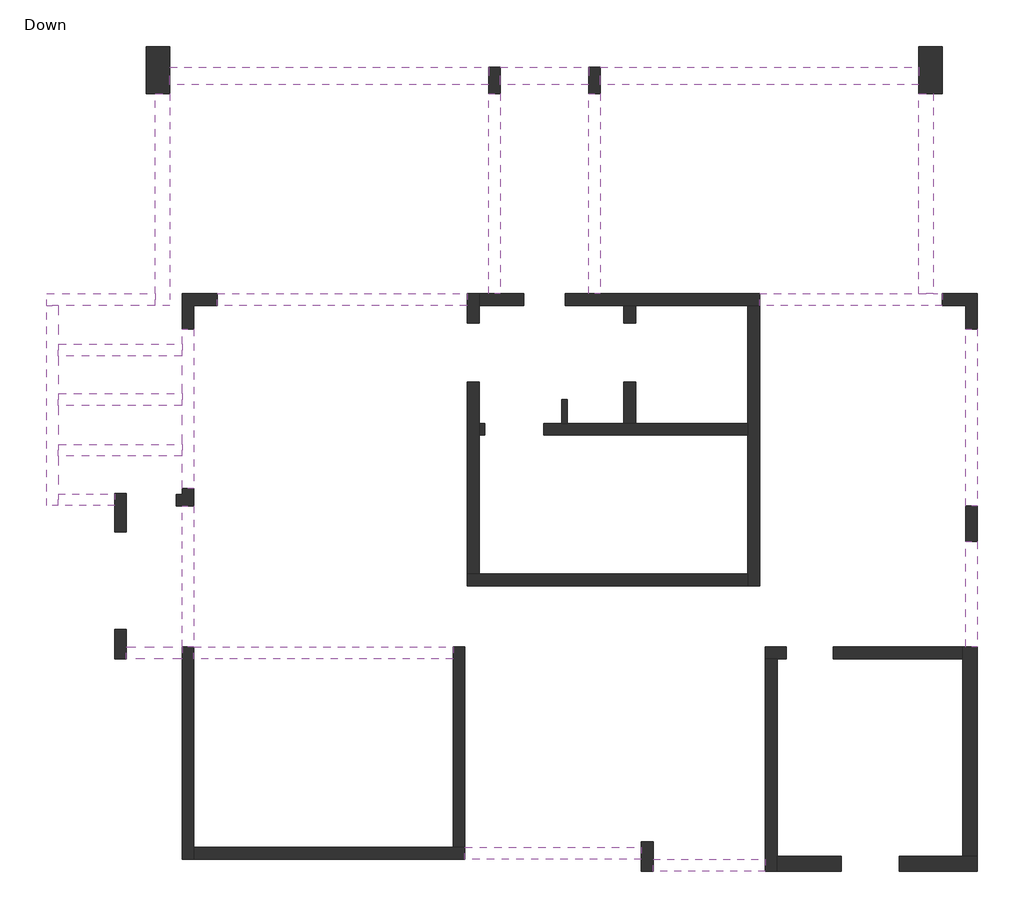
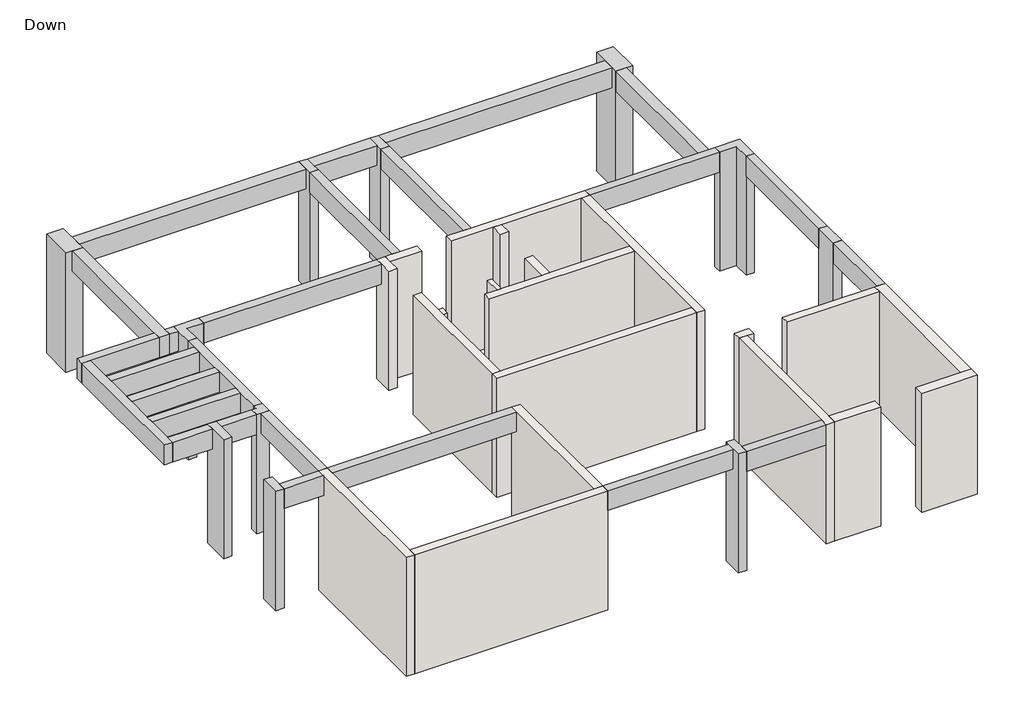
# One storey: 23 beams, 20 walls, 11 columns.
"""IFC4 building model written with IfcOpenShell, lengths in millimetres."""

from ifc_helpers import new_model, si_unit, frame, origin, origin_with_axes, place, context, project, spatial, polyline, outline, extrude, faceted_brep, element, save

model = new_model("IFC4")

# Units and contexts
model_context = context("Model", 3, world=origin())
ifc_project = project(units=[si_unit("LENGTHUNIT", "METRE", prefix="MILLI")], contexts=[model_context])

# Site, building, storey
site = spatial("IfcSite", under=ifc_project)
building = spatial("IfcBuilding", under=site)
storey = spatial("IfcBuildingStorey", under=building, Name="Down", Elevation=0.0)

# Beams
placement = place(None, origin())
element("IfcBeam", 1, ObjectType="Concrete Rectengular Beam : 20/50", at=placement, inside=storey, context=model_context, shape_type="Brep", body=[
    faceted_brep([(-4636.0027125, 7405.5532536, 3000.0), (-4636.0027125, 7605.5532536, 3000.0), (-8876.8844551, 7605.5532536, 3000.0), (-8876.8844551, 7405.5532536, 3000.0), (-4636.0027125, 7405.5532536, 2500.0), (-4636.0027125, 7405.5532536, 2850.0), (-8876.8844551, 7405.5532536, 2500.0), (-4636.0027125, 7605.5532536, 2500.0), (-8876.8844551, 7605.5532536, 2500.0)], [[[0, 1, 2, 3]], [[4, 5, 0, 3, 6]], [[7, 4, 6, 8]], [[1, 7, 8, 2]], [[1, 0, 5, 4, 7]], [[3, 2, 8, 6]]]),
])
element("IfcBeam", 2, ObjectType="Concrete Rectengular Beam : 20/50", at=placement, inside=storey, context=model_context, shape_type="Brep", body=[
    faceted_brep([(3423.240421, 7405.5532536, 3000.0), (3423.240421, 7605.5532536, 3000.0), (3276.9297982, 7605.5532536, 3000.0), (3026.9297982, 7605.5532536, 3000.0), (323.9972875, 7605.5532536, 3000.0), (323.9972875, 7405.5532536, 3000.0), (3423.240421, 7605.5532536, 2500.0), (3276.9297982, 7605.5532536, 2500.0), (3026.9297982, 7605.5532536, 2500.0), (323.9972875, 7605.5532536, 2500.0), (3423.240421, 7405.5532536, 2500.0), (323.9972875, 7405.5532536, 2500.0), (323.9972875, 7405.5532536, 2850.0)], [[[0, 1, 2, 3, 4, 5]], [[1, 6, 7, 8, 9, 4, 3, 2]], [[6, 10, 11, 9, 8, 7]], [[10, 0, 5, 12, 11]], [[1, 0, 10, 6]], [[5, 4, 9, 11, 12]]]),
])
element("IfcBeam", 3, ObjectType="Concrete Rectengular Beam : 20/50", at=placement, inside=storey, context=model_context, shape_type="Brep", body=[
    faceted_brep([(-9277.1472957, 1603.8855607, 3000.0), (-9277.1472957, 1403.8855607, 3000.0), (-4877.1268931, 1403.8855607, 3000.0), (-4877.1268931, 1603.8855607, 3000.0), (-9276.8844551, 1603.8855607, 3000.0), (-9277.1472957, 1603.8855607, 2500.0), (-4877.1268931, 1603.8855607, 2850.0), (-4877.1268931, 1603.8855607, 2500.0), (-9276.8844551, 1603.8855607, 2500.0), (-9277.1472957, 1403.8855607, 2500.0), (-4877.1268931, 1403.8855607, 2500.0), (-9277.1472957, 1403.8855607, 2850.0), (-4877.1268931, 1403.8855607, 2850.0)], [[[0, 1, 2, 3, 4]], [[5, 0, 4, 3, 6, 7, 8]], [[9, 5, 8, 7, 10]], [[1, 11, 9, 10, 12, 2]], [[1, 0, 5, 9, 11]], [[3, 2, 12, 10, 7, 6]]]),
])
element("IfcBeam", 4, ObjectType="Concrete Rectengular Beam : 20/50", at=placement, inside=storey, context=model_context, shape_type="Brep", body=[
    faceted_brep([(-9276.8844551, 3997.7532903, 3000.0), (-9476.8844551, 3997.7532903, 3000.0), (-9476.8844551, 1603.8855607, 3000.0), (-9277.1472957, 1603.8855607, 3000.0), (-9276.8844551, 1603.8855607, 3000.0), (-9276.8844551, 3997.7532903, 2500.0), (-9276.8844551, 1603.8855607, 2850.0), (-9276.8844551, 1603.8855607, 2500.0), (-9476.8844551, 3997.7532903, 2500.0), (-9277.1472957, 1603.8855607, 2500.0), (-9476.8844551, 1603.8855607, 2500.0), (-9476.8844551, 3997.7532903, 2850.0), (-9476.8844551, 1603.8855607, 2850.0)], [[[0, 1, 2, 3, 4]], [[5, 0, 4, 6, 7]], [[8, 5, 7, 9, 10]], [[1, 11, 8, 10, 12, 2]], [[1, 0, 5, 8, 11]], [[4, 3, 2, 12, 10, 9, 7, 6]]]),
])
element("IfcBeam", 5, ObjectType="Concrete Rectengular Beam : 20/50", at=placement, inside=storey, context=model_context, shape_type="Brep", body=[
    faceted_brep([(-9276.8844551, 7005.5532536, 3000.0), (-9476.8844551, 7005.5532536, 3000.0), (-9476.8844551, 6745.5532536, 3000.0), (-9476.8844551, 6545.5532536, 3000.0), (-9476.8844551, 5905.5532536, 3000.0), (-9476.8844551, 5705.5532536, 3000.0), (-9476.8844551, 5045.5532536, 3000.0), (-9476.8844551, 4845.5532536, 3000.0), (-9476.8844551, 4297.7532903, 3000.0), (-9276.8844551, 4297.7532903, 3000.0), (-9276.8844551, 7005.5532536, 2500.0), (-9276.8844551, 4297.7532903, 2500.0), (-9476.8844551, 7005.5532536, 2500.0), (-9476.8844551, 4297.7532903, 2500.0), (-9476.8844551, 4845.5532536, 2500.0), (-9476.8844551, 5045.5532536, 2500.0), (-9476.8844551, 5705.5532536, 2500.0), (-9476.8844551, 5905.5532536, 2500.0), (-9476.8844551, 6545.5532536, 2500.0), (-9476.8844551, 6745.5532536, 2500.0)], [[[0, 1, 2, 3, 4, 5, 6, 7, 8, 9]], [[10, 0, 9, 11]], [[12, 10, 11, 13, 14, 15, 16, 17, 18, 19]], [[1, 12, 19, 18, 17, 16, 15, 14, 13, 8, 7, 6, 5, 4, 3, 2]], [[1, 0, 10, 12]], [[9, 8, 13, 11]]]),
])
element("IfcBeam", 6, ObjectType="Concrete Rectengular Beam : 20/50", at=placement, inside=storey, context=model_context, shape_type="Brep", body=[
    faceted_brep([(-1681.0647566, -1997.4530794, 3000.0), (-1681.0647566, -1797.4530794, 3000.0), (-4677.1268931, -1797.4530794, 3000.0), (-4677.1268931, -1997.4530794, 3000.0), (-1681.0647566, -1997.4530794, 2500.0), (-4677.1268931, -1997.4530794, 2500.0), (-1681.0647566, -1797.4530794, 2500.0), (-4677.1268931, -1797.4530794, 2500.0), (-1681.0647566, -1797.4530794, 2850.0), (-4677.1268931, -1797.4530794, 2850.0)], [[[0, 1, 2, 3]], [[4, 0, 3, 5]], [[6, 4, 5, 7]], [[2, 1, 8, 6, 7, 9]], [[1, 0, 4, 6, 8]], [[3, 2, 9, 7, 5]]]),
])
element("IfcBeam", 7, ObjectType="Concrete Rectengular Beam : 20/50", at=placement, inside=storey, context=model_context, shape_type="Brep", body=[
    faceted_brep([(-1481.0647566, -2001.586272, 3000.0), (-1481.0647566, -2201.586272, 3000.0), (423.0052446, -2201.586272, 3000.0), (423.0052446, -2001.586272, 3000.0), (-1481.0647566, -2201.586272, 2500.0), (423.0052446, -2201.586272, 2500.0), (-1481.0647566, -2001.586272, 2500.0), (423.0052446, -2001.586272, 2500.0), (-1481.0647566, -2001.586272, 2850.0), (423.0052446, -2001.586272, 2850.0)], [[[0, 1, 2, 3]], [[1, 4, 5, 2]], [[4, 6, 7, 5]], [[6, 8, 0, 3, 9, 7]], [[1, 0, 8, 6, 4]], [[3, 2, 5, 7, 9]]]),
])
element("IfcBeam", 8, ObjectType="Concrete Rectengular Beam : 20/50", at=placement, inside=storey, context=model_context, shape_type="Brep", body=[
    faceted_brep([(4023.240421, 3398.9311809, 3000.0), (3823.240421, 3398.9311809, 3000.0), (3823.240421, 1603.8858088, 3000.0), (4023.240421, 1603.8858088, 3000.0), (4023.240421, 3398.9311809, 2500.0), (4023.240421, 1603.8858088, 2500.0), (3823.240421, 3398.9311809, 2500.0), (3823.240421, 1603.8858088, 2500.0), (3823.240421, 1603.8858088, 2850.0)], [[[0, 1, 2, 3]], [[4, 0, 3, 5]], [[6, 4, 5, 7]], [[1, 6, 7, 8, 2]], [[1, 0, 4, 6]], [[3, 2, 8, 7, 5]]]),
])
element("IfcBeam", 9, ObjectType="Concrete Rectengular Beam : 20/50", at=placement, inside=storey, context=model_context, shape_type="SweptSolid", body=[
    extrude(outline(polyline([(3823.240421, 7005.5532536), (4023.240421, 7005.5532536), (4023.240421, 3998.9311809), (3823.240421, 3998.9311809), (3823.240421, 7005.5532536)])), frame((0.0, 0.0, 2500.0), z_axis=(0.0, 0.0, 1.0), x_axis=(1.0, 0.0, 0.0)), (0.0, 0.0, 1.0), 500.0),
])
element("IfcBeam", 10, ObjectType="Concrete Rectengular Beam : 20/50", at=placement, inside=storey, context=model_context, shape_type="Brep", body=[
    faceted_brep([(-2375.600893, 11003.3317688, 3000.0), (-2575.600893, 11003.3317688, 3000.0), (-2575.600893, 7605.5532536, 3000.0), (-2375.600893, 7605.5532536, 3000.0), (-2575.600893, 11003.3317688, 2500.0), (-2575.600893, 7605.5532536, 2500.0), (-2575.600893, 7605.5532536, 2850.0), (-2375.600893, 11003.3317688, 2500.0), (-2375.600893, 7605.5532536, 2500.0), (-2375.600893, 7605.5532536, 2850.0)], [[[0, 1, 2, 3]], [[1, 4, 5, 6, 2]], [[4, 7, 8, 5]], [[7, 0, 3, 9, 8]], [[1, 0, 7, 4]], [[3, 2, 6, 5, 8, 9]]]),
])
element("IfcBeam", 11, ObjectType="Concrete Rectengular Beam : 20/50", at=placement, inside=storey, context=model_context, shape_type="Brep", body=[
    faceted_brep([(-4072.3731245, 11003.3317688, 3000.0), (-4272.3731245, 11003.3317688, 3000.0), (-4272.3731245, 7605.5532536, 3000.0), (-4072.3731245, 7605.5532536, 3000.0), (-4072.3731245, 11003.3317688, 2500.0), (-4072.3731245, 7605.5532536, 2850.0), (-4072.3731245, 7605.5532536, 2500.0), (-4272.3731245, 11003.3317688, 2500.0), (-4272.3731245, 7605.5532536, 2500.0), (-4272.3731245, 7605.5532536, 2850.0)], [[[0, 1, 2, 3]], [[4, 0, 3, 5, 6]], [[7, 4, 6, 8]], [[1, 7, 8, 9, 2]], [[1, 0, 4, 7]], [[3, 2, 9, 8, 6, 5]]]),
])
element("IfcBeam", 12, ObjectType="Concrete Rectengular Beam : 20/50", at=placement, inside=storey, context=model_context, shape_type="Brep", body=[
    faceted_brep([(-9476.8844551, 7405.5532536, 3000.0), (-9476.8844551, 7605.5532536, 3000.0), (-9682.6961091, 7605.5532536, 3000.0), (-9682.6961091, 7405.5532536, 3000.0), (-9476.8844551, 7605.5532536, 2500.0), (-9682.6961091, 7605.5532536, 2500.0), (-9682.6961091, 7605.5532536, 2850.0), (-9476.8844551, 7405.5532536, 2500.0), (-9682.6961091, 7405.5532536, 2500.0), (-9476.8844551, 7405.5532536, 2850.0)], [[[0, 1, 2, 3]], [[1, 4, 5, 6, 2]], [[4, 7, 8, 5]], [[7, 9, 0, 3, 8]], [[1, 0, 9, 7, 4]], [[3, 2, 6, 5, 8]]]),
    faceted_brep([(-11776.8844551, 7405.5532536, 3000.0), (-11776.8844551, 7605.5532536, 3000.0), (-11776.8844551, 7605.5532536, 2500.0), (-11776.8844551, 7405.5532536, 2500.0), (-9932.6961091, 7605.5532536, 3000.0), (-9932.6961091, 7405.5532536, 3000.0), (-9932.6961091, 7405.5532536, 2500.0), (-9932.6961091, 7605.5532536, 2500.0), (-11576.8844551, 7405.5532536, 3000.0), (-11576.8844551, 7405.5532536, 2500.0)], [[[0, 1, 2, 3]], [[4, 5, 6, 7]], [[1, 0, 8, 5, 4]], [[2, 1, 4, 7]], [[3, 2, 7, 6, 9]], [[0, 3, 9, 6, 5, 8]]]),
])
element("IfcBeam", 13, ObjectType="Concrete Rectengular Beam : 20/50", at=placement, inside=storey, context=model_context, shape_type="Brep", body=[
    faceted_brep([(-11776.8844551, 4005.5532536, 3000.0), (-11576.8844551, 4005.5532536, 3000.0), (-11576.8844551, 4205.5532536, 3000.0), (-11576.8844551, 4845.5532536, 3000.0), (-11576.8844551, 5045.5532536, 3000.0), (-11576.8844551, 5705.5532536, 3000.0), (-11576.8844551, 5905.5532536, 3000.0), (-11576.8844551, 6545.5532536, 3000.0), (-11576.8844551, 6745.5532536, 3000.0), (-11576.8844551, 7405.5532536, 3000.0), (-11776.8844551, 7405.5532536, 3000.0), (-11776.8844551, 4005.5532536, 2500.0), (-11776.8844551, 7405.5532536, 2500.0), (-11576.8844551, 4005.5532536, 2500.0), (-11576.8844551, 7405.5532536, 2500.0), (-11576.8844551, 6745.5532536, 2500.0), (-11576.8844551, 6545.5532536, 2500.0), (-11576.8844551, 5905.5532536, 2500.0), (-11576.8844551, 5705.5532536, 2500.0), (-11576.8844551, 5045.5532536, 2500.0), (-11576.8844551, 4845.5532536, 2500.0), (-11576.8844551, 4205.5532536, 2500.0), (-11576.8844551, 7405.5532536, 2850.0)], [[[0, 1, 2, 3, 4, 5, 6, 7, 8, 9, 10]], [[11, 0, 10, 12]], [[13, 11, 12, 14, 15, 16, 17, 18, 19, 20, 21]], [[1, 13, 21, 20, 19, 18, 17, 16, 15, 14, 22, 9, 8, 7, 6, 5, 4, 3, 2]], [[10, 9, 22, 14, 12]], [[1, 0, 11, 13]]]),
])
element("IfcBeam", 14, ObjectType="Concrete Rectengular Beam : 20/50", at=placement, inside=storey, context=model_context, shape_type="Brep", body=[
    faceted_brep([(-9576.8844551, 4005.5532536, 3000.0), (-9576.8844551, 4197.7532903, 3000.0), (-9476.8844551, 4197.7532903, 3000.0), (-9476.8844551, 4205.5532536, 3000.0), (-10423.025528, 4205.5532536, 3000.0), (-10423.025528, 4005.5532536, 3000.0), (-9576.8844551, 4005.5532536, 2500.0), (-9576.8844551, 4005.5532536, 2850.0), (-10423.025528, 4005.5532536, 2850.0), (-10423.025528, 4005.5532536, 2500.0), (-9576.8844551, 4197.7532903, 2500.0), (-10423.025528, 4205.5532536, 2500.0), (-9476.8844551, 4205.5532536, 2500.0), (-9476.8844551, 4197.7532903, 2500.0), (-9476.8844551, 4205.5532536, 2850.0), (-10423.025528, 4205.5532536, 2850.0)], [[[0, 1, 2, 3, 4, 5]], [[6, 7, 0, 5, 8, 9]], [[10, 6, 9, 11, 12, 13]], [[3, 14, 12, 11, 15, 4]], [[10, 1, 0, 7, 6]], [[1, 10, 13, 2]], [[2, 13, 12, 14, 3]], [[5, 4, 15, 11, 9, 8]]]),
    faceted_brep([(-11576.8844551, 4005.5532536, 3000.0), (-11576.8844551, 4205.5532536, 3000.0), (-11576.8844551, 4205.5532536, 2850.0), (-11576.8844551, 4205.5532536, 2500.0), (-11576.8844551, 4005.5532536, 2500.0), (-10623.025528, 4205.5532536, 3000.0), (-10623.025528, 4005.5532536, 3000.0), (-10623.025528, 4005.5532536, 2500.0), (-10623.025528, 4205.5532536, 2500.0), (-10623.025528, 4205.5532536, 2850.0)], [[[0, 1, 2, 3, 4]], [[5, 6, 7, 8, 9]], [[1, 0, 6, 5]], [[0, 4, 7, 6]], [[4, 3, 8, 7]], [[3, 2, 1, 5, 9, 8]]]),
])
element("IfcBeam", 15, ObjectType="Concrete Rectengular Beam : 20/50", at=placement, inside=storey, context=model_context, shape_type="Brep", body=[
    faceted_brep([(-9476.8844551, 4845.5532536, 3000.0), (-9476.8844551, 5045.5532536, 3000.0), (-11576.8844551, 5045.5532536, 3000.0), (-11576.8844551, 4845.5532536, 3000.0), (-9476.8844551, 5045.5532536, 2850.0), (-9476.8844551, 5045.5532536, 2500.0), (-11576.8844551, 5045.5532536, 2500.0), (-11576.8844551, 5045.5532536, 2850.0), (-9476.8844551, 4845.5532536, 2500.0), (-11576.8844551, 4845.5532536, 2500.0), (-9476.8844551, 4845.5532536, 2850.0), (-11576.8844551, 4845.5532536, 2850.0)], [[[0, 1, 2, 3]], [[1, 4, 5, 6, 7, 2]], [[5, 8, 9, 6]], [[8, 10, 0, 3, 11, 9]], [[1, 0, 10, 8, 5, 4]], [[3, 2, 7, 6, 9, 11]]]),
])
element("IfcBeam", 16, ObjectType="Concrete Rectengular Beam : 20/50", at=placement, inside=storey, context=model_context, shape_type="Brep", body=[
    faceted_brep([(-9476.8844551, 5705.5532536, 3000.0), (-9476.8844551, 5905.5532536, 3000.0), (-11576.8844551, 5905.5532536, 3000.0), (-11576.8844551, 5705.5532536, 3000.0), (-9476.8844551, 5905.5532536, 2850.0), (-9476.8844551, 5905.5532536, 2500.0), (-11576.8844551, 5905.5532536, 2500.0), (-11576.8844551, 5905.5532536, 2850.0), (-9476.8844551, 5705.5532536, 2500.0), (-11576.8844551, 5705.5532536, 2500.0), (-9476.8844551, 5705.5532536, 2850.0), (-11576.8844551, 5705.5532536, 2850.0)], [[[0, 1, 2, 3]], [[1, 4, 5, 6, 7, 2]], [[5, 8, 9, 6]], [[8, 10, 0, 3, 11, 9]], [[1, 0, 10, 8, 5, 4]], [[3, 2, 7, 6, 9, 11]]]),
])
element("IfcBeam", 17, ObjectType="Concrete Rectengular Beam : 20/50", at=placement, inside=storey, context=model_context, shape_type="Brep", body=[
    faceted_brep([(-9476.8844551, 6545.5532536, 3000.0), (-9476.8844551, 6745.5532536, 3000.0), (-11576.8844551, 6745.5532536, 3000.0), (-11576.8844551, 6545.5532536, 3000.0), (-9476.8844551, 6745.5532536, 2850.0), (-9476.8844551, 6745.5532536, 2500.0), (-11576.8844551, 6745.5532536, 2500.0), (-11576.8844551, 6745.5532536, 2850.0), (-9476.8844551, 6545.5532536, 2500.0), (-11576.8844551, 6545.5532536, 2500.0), (-9476.8844551, 6545.5532536, 2850.0), (-11576.8844551, 6545.5532536, 2850.0)], [[[0, 1, 2, 3]], [[1, 4, 5, 6, 7, 2]], [[5, 8, 9, 6]], [[8, 10, 0, 3, 11, 9]], [[1, 0, 10, 8, 5, 4]], [[3, 2, 7, 6, 9, 11]]]),
])
element("IfcBeam", 18, ObjectType="Concrete Rectengular Beam : 20/50", at=placement, inside=storey, context=model_context, shape_type="Brep", body=[
    faceted_brep([(-10423.025528, 1603.8855607, 3000.0), (-10423.025528, 1403.8855607, 3000.0), (-9477.1472957, 1403.8855607, 3000.0), (-9477.1472957, 1603.8855607, 3000.0), (-10423.025528, 1603.8855607, 2500.0), (-10423.025528, 1603.8855607, 2850.0), (-9477.1472957, 1603.8855607, 2500.0), (-10423.025528, 1403.8855607, 2500.0), (-9477.1472957, 1403.8855607, 2500.0)], [[[0, 1, 2, 3]], [[4, 5, 0, 3, 6]], [[7, 4, 6, 8]], [[1, 7, 8, 2]], [[1, 0, 5, 4, 7]], [[3, 2, 8, 6]]]),
])
element("IfcBeam", 19, ObjectType="Concrete Rectengular Beam : 25/50", at=placement, inside=storey, context=model_context, shape_type="Brep", body=[
    faceted_brep([(3276.9297982, 11001.5732233, 3000.0), (3026.9297982, 11001.5732233, 3000.0), (3026.9297982, 7605.5532536, 3000.0), (3276.9297982, 7605.5532536, 3000.0), (3276.9297982, 11001.5732233, 2500.0), (3276.9297982, 7605.5532536, 2500.0), (3026.9297982, 11001.5732233, 2500.0), (3026.9297982, 7605.5532536, 2500.0), (3026.9297982, 7605.5532536, 2850.0)], [[[0, 1, 2, 3]], [[4, 0, 3, 5]], [[6, 4, 5, 7]], [[1, 6, 7, 8, 2]], [[1, 0, 4, 6]], [[3, 2, 8, 7, 5]]]),
])
element("IfcBeam", 20, ObjectType="Concrete Rectengular Beam : 25/50", at=placement, inside=storey, context=model_context, shape_type="Brep", body=[
    faceted_brep([(-9932.6961091, 7405.5532536, 3000.0), (-9682.6961091, 7405.5532536, 3000.0), (-9682.6961091, 7605.5532536, 3000.0), (-9682.6961091, 11001.5732233, 3000.0), (-9932.6961091, 11001.5732233, 3000.0), (-9932.6961091, 7605.5532536, 3000.0), (-9682.6961091, 7405.5532536, 2500.0), (-9682.6961091, 7605.5532536, 2500.0), (-9682.6961091, 11001.5732233, 2500.0), (-9932.6961091, 7405.5532536, 2500.0), (-9932.6961091, 7605.5532536, 2500.0), (-9932.6961091, 11001.5732233, 2500.0)], [[[0, 1, 2, 3, 4, 5]], [[1, 6, 7, 8, 3, 2]], [[6, 9, 10, 11, 8, 7]], [[9, 0, 5, 4, 11, 10]], [[4, 3, 8, 11]], [[1, 0, 9, 6]]]),
])
element("IfcBeam", 21, ObjectType="Concrete Rectengular Beam : 30/50", at=placement, inside=storey, context=model_context, shape_type="Brep", body=[
    faceted_brep([(-9682.6961091, 11451.9234339, 3000.0), (-9682.6961091, 11151.9234339, 3000.0), (-4272.3731245, 11151.9234339, 3000.0), (-4272.3731245, 11451.9234339, 3000.0), (-9682.6961091, 11451.9234339, 2500.0), (-4272.3731245, 11451.9234339, 2500.0), (-9682.6961091, 11151.9234339, 2500.0), (-4272.3731245, 11151.9234339, 2500.0), (-9682.6961091, 11151.9234339, 2850.0), (-4272.3731245, 11151.9234339, 2850.0)], [[[0, 1, 2, 3]], [[4, 0, 3, 5]], [[6, 4, 5, 7]], [[1, 8, 6, 7, 9, 2]], [[1, 0, 4, 6, 8]], [[3, 2, 9, 7, 5]]]),
])
element("IfcBeam", 22, ObjectType="Concrete Rectengular Beam : 30/50", at=placement, inside=storey, context=model_context, shape_type="Brep", body=[
    faceted_brep([(-2575.600893, 11151.9234339, 3000.0), (-2575.600893, 11451.9234339, 3000.0), (-4072.3731245, 11451.9234339, 3000.0), (-4072.3731245, 11151.9234339, 3000.0), (-2575.600893, 11151.9234339, 2500.0), (-2575.600893, 11151.9234339, 2850.0), (-4072.3731245, 11151.9234339, 2850.0), (-4072.3731245, 11151.9234339, 2500.0), (-2575.600893, 11451.9234339, 2500.0), (-4072.3731245, 11451.9234339, 2500.0)], [[[0, 1, 2, 3]], [[4, 5, 0, 3, 6, 7]], [[8, 4, 7, 9]], [[1, 8, 9, 2]], [[1, 0, 5, 4, 8]], [[3, 2, 9, 7, 6]]]),
])
element("IfcBeam", 23, ObjectType="Concrete Rectengular Beam : 30/50", at=placement, inside=storey, context=model_context, shape_type="Brep", body=[
    faceted_brep([(3026.9297982, 11151.9234339, 3000.0), (3026.9297982, 11451.9234339, 3000.0), (-2375.600893, 11451.9234339, 3000.0), (-2375.600893, 11151.9234339, 3000.0), (3026.9297982, 11151.9234339, 2500.0), (3026.9297982, 11151.9234339, 2850.0), (-2375.600893, 11151.9234339, 2850.0), (-2375.600893, 11151.9234339, 2500.0), (3026.9297982, 11451.9234339, 2500.0), (-2375.600893, 11451.9234339, 2500.0)], [[[0, 1, 2, 3]], [[4, 5, 0, 3, 6, 7]], [[8, 4, 7, 9]], [[1, 8, 9, 2]], [[1, 0, 5, 4, 8]], [[3, 2, 9, 7, 6]]]),
])

# Columns
element("IfcColumn", 24, ObjectType="Concrete Rectengular Column : 20/45", at=placement, inside=storey, context=model_context, shape_type="Brep", body=[
    faceted_brep([(-2375.600893, 11453.3317688, 0.0), (-2375.600893, 11003.3317688, 0.0), (-2575.600893, 11003.3317688, 0.0), (-2575.600893, 11453.3317688, 0.0), (-2375.600893, 11453.3317688, 3000.0), (-2375.600893, 11151.9234339, 3000.0), (-2375.600893, 11003.3317688, 3000.0), (-2575.600893, 11003.3317688, 3000.0), (-2575.600893, 11151.9234339, 3000.0), (-2575.600893, 11453.3317688, 3000.0)], [[[0, 1, 2, 3]], [[4, 5, 6, 1, 0]], [[6, 7, 2, 1]], [[7, 8, 9, 3, 2]], [[9, 4, 0, 3]], [[4, 9, 8, 7, 6, 5]]]),
])
element("IfcColumn", 25, ObjectType="Concrete Rectengular Column : 20/45", at=placement, inside=storey, context=model_context, shape_type="Brep", body=[
    faceted_brep([(-4072.3731245, 11453.3317688, 0.0), (-4072.3731245, 11003.3317688, 0.0), (-4272.3731245, 11003.3317688, 0.0), (-4272.3731245, 11453.3317688, 0.0), (-4072.3731245, 11453.3317688, 3000.0), (-4072.3731245, 11151.9234339, 3000.0), (-4072.3731245, 11003.3317688, 3000.0), (-4272.3731245, 11003.3317688, 3000.0), (-4272.3731245, 11151.9234339, 3000.0), (-4272.3731245, 11453.3317688, 3000.0)], [[[0, 1, 2, 3]], [[4, 5, 6, 1, 0]], [[6, 7, 2, 1]], [[7, 8, 9, 3, 2]], [[9, 4, 0, 3]], [[4, 9, 8, 7, 6, 5]]]),
])
element("IfcColumn", 26, ObjectType="Concrete Rectengular Column : 20/50", at=placement, inside=storey, context=model_context, shape_type="Brep", body=[
    faceted_brep([(-10423.025528, 1900.4395709, 0.0), (-10423.025528, 1400.4395709, 0.0), (-10623.025528, 1400.4395709, 0.0), (-10623.025528, 1900.4395709, 0.0), (-10423.025528, 1900.4395709, 3000.0), (-10423.025528, 1603.8855607, 3000.0), (-10423.025528, 1400.4395709, 3000.0), (-10423.025528, 1900.4395709, 2850.0), (-10623.025528, 1400.4395709, 3000.0), (-10623.025528, 1900.4395709, 3000.0), (-10623.025528, 1900.4395709, 2850.0)], [[[0, 1, 2, 3]], [[4, 5, 6, 1, 0, 7]], [[6, 8, 2, 1]], [[8, 9, 10, 3, 2]], [[9, 4, 7, 0, 3, 10]], [[4, 9, 8, 6, 5]]]),
])
element("IfcColumn", 27, ObjectType="Concrete Rectengular Column : 20/50", at=placement, inside=storey, context=model_context, shape_type="Brep", body=[
    faceted_brep([(-1481.0647566, -1701.586272, 0.0), (-1481.0647566, -2201.586272, 0.0), (-1681.0647566, -2201.586272, 0.0), (-1681.0647566, -1701.586272, 0.0), (-1481.0647566, -1701.586272, 3000.0), (-1481.0647566, -2001.586272, 3000.0), (-1481.0647566, -2201.586272, 3000.0), (-1481.0647566, -1701.586272, 2850.0), (-1681.0647566, -2201.586272, 3000.0), (-1681.0647566, -1797.4530794, 3000.0), (-1681.0647566, -1701.586272, 3000.0), (-1681.0647566, -1701.586272, 2850.0)], [[[0, 1, 2, 3]], [[4, 5, 6, 1, 0, 7]], [[6, 8, 2, 1]], [[8, 9, 10, 11, 3, 2]], [[10, 4, 7, 0, 3, 11]], [[4, 10, 9, 8, 6, 5]]]),
])
element("IfcColumn", 28, ObjectType="Concrete Rectengular Column : 20/60", at=placement, inside=storey, context=model_context, shape_type="SweptSolid", body=[
    extrude(outline(polyline([(4023.240421, 3998.9311809), (4023.240421, 3398.9311809), (3823.240421, 3398.9311809), (3823.240421, 3998.9311809), (4023.240421, 3998.9311809)])), origin_with_axes(), (0.0, 0.0, 1.0), 3000.0),
])
element("IfcColumn", 29, ObjectType="Concrete Rectengular Column : 20/65", at=placement, inside=storey, context=model_context, shape_type="Brep", body=[
    faceted_brep([(-10423.025528, 4208.1905626, 0.0), (-10423.025528, 3558.1905626, 0.0), (-10623.025528, 3558.1905626, 0.0), (-10623.025528, 4208.1905626, 0.0), (-10423.025528, 4208.1905626, 3000.0), (-10423.025528, 4205.5532536, 3000.0), (-10423.025528, 4005.5532536, 3000.0), (-10423.025528, 3558.1905626, 3000.0), (-10423.025528, 3558.1905626, 2850.0), (-10423.025528, 4208.1905626, 2850.0), (-10623.025528, 3558.1905626, 3000.0), (-10623.025528, 3558.1905626, 2850.0), (-10623.025528, 4005.5532536, 3000.0), (-10623.025528, 4205.5532536, 3000.0), (-10623.025528, 4208.1905626, 3000.0), (-10623.025528, 4208.1905626, 2850.0)], [[[0, 1, 2, 3]], [[4, 5, 6, 7, 8, 1, 0, 9]], [[7, 10, 11, 2, 1, 8]], [[10, 12, 13, 14, 15, 3, 2, 11]], [[14, 4, 9, 0, 3, 15]], [[4, 14, 13, 12, 10, 7, 6, 5]]]),
])
element("IfcColumn", 30, ObjectType="Concrete Rectengular Column : 40/80", at=placement, inside=storey, context=model_context, shape_type="Brep", body=[
    faceted_brep([(3426.9297982, 11801.5732233, 0.0), (3426.9297982, 11001.5732233, 0.0), (3026.9297982, 11001.5732233, 0.0), (3026.9297982, 11801.5732233, 0.0), (3426.9297982, 11801.5732233, 3000.0), (3426.9297982, 11001.5732233, 3000.0), (3026.9297982, 11001.5732233, 3000.0), (3026.9297982, 11151.9234339, 3000.0), (3026.9297982, 11801.5732233, 3000.0)], [[[0, 1, 2, 3]], [[4, 5, 1, 0]], [[5, 6, 2, 1]], [[6, 7, 8, 3, 2]], [[8, 4, 0, 3]], [[4, 8, 7, 6, 5]]]),
])
element("IfcColumn", 31, ObjectType="Concrete Rectengular Column : 40/80", at=placement, inside=storey, context=model_context, shape_type="Brep", body=[
    faceted_brep([(-9682.6961091, 11801.5732233, 0.0), (-9682.6961091, 11001.5732233, 0.0), (-10082.6961091, 11001.5732233, 0.0), (-10082.6961091, 11801.5732233, 0.0), (-9682.6961091, 11801.5732233, 3000.0), (-9682.6961091, 11151.9234339, 3000.0), (-9682.6961091, 11001.5732233, 3000.0), (-10082.6961091, 11001.5732233, 3000.0), (-10082.6961091, 11801.5732233, 3000.0)], [[[0, 1, 2, 3]], [[4, 5, 6, 1, 0]], [[6, 7, 2, 1]], [[7, 8, 3, 2]], [[8, 4, 0, 3]], [[4, 8, 7, 6, 5]]]),
])
element("IfcColumn", 32, ObjectType="L Column : 30/30/20/20", at=placement, inside=storey, context=model_context, shape_type="Brep", body=[
    faceted_brep([(-9276.8844551, 3997.7532903, 0.0), (-9576.8844551, 3997.7532903, 0.0), (-9576.8844551, 4197.7532903, 0.0), (-9476.8844551, 4197.7532903, 0.0), (-9476.8844551, 4297.7532903, 0.0), (-9276.8844551, 4297.7532903, 0.0), (-9276.8844551, 3997.7532903, 3000.0), (-9476.8844551, 3997.7532903, 3000.0), (-9576.8844551, 3997.7532903, 3000.0), (-9576.8844551, 3997.7532903, 2850.0), (-9576.8844551, 4005.5532536, 3000.0), (-9576.8844551, 4197.7532903, 3000.0), (-9476.8844551, 4197.7532903, 3000.0), (-9476.8844551, 4205.5532536, 3000.0), (-9476.8844551, 4297.7532903, 3000.0), (-9276.8844551, 4297.7532903, 3000.0)], [[[0, 1, 2, 3, 4, 5]], [[6, 7, 8, 9, 1, 0]], [[8, 10, 11, 2, 1, 9]], [[11, 12, 3, 2]], [[12, 13, 14, 4, 3]], [[14, 15, 5, 4]], [[15, 6, 0, 5]], [[6, 15, 14, 13, 12, 11, 10, 8, 7]]]),
])
element("IfcColumn", 33, ObjectType="L Column : 60/60/20/20", at=placement, inside=storey, context=model_context, shape_type="Brep", body=[
    faceted_brep([(4023.240421, 7605.5532536, 0.0), (4023.240421, 7005.5532536, 0.0), (3823.240421, 7005.5532536, 0.0), (3823.240421, 7405.5532536, 0.0), (3423.240421, 7405.5532536, 0.0), (3423.240421, 7605.5532536, 0.0), (4023.240421, 7605.5532536, 3000.0), (4023.240421, 7005.5532536, 3000.0), (3823.240421, 7005.5532536, 3000.0), (3823.240421, 7405.5532536, 3000.0), (3823.240421, 7405.5532536, 2850.0), (3423.240421, 7405.5532536, 3000.0), (3423.240421, 7605.5532536, 3000.0)], [[[0, 1, 2, 3, 4, 5]], [[6, 7, 1, 0]], [[7, 8, 2, 1]], [[8, 9, 10, 3, 2]], [[9, 11, 4, 3, 10]], [[11, 12, 5, 4]], [[12, 6, 0, 5]], [[6, 12, 11, 9, 8, 7]]]),
])
element("IfcColumn", 34, ObjectType="L Column : 60/60/20/20", at=placement, inside=storey, context=model_context, shape_type="Brep", body=[
    faceted_brep([(-9476.8844551, 7605.5532536, 0.0), (-8876.8844551, 7605.5532536, 0.0), (-8876.8844551, 7405.5532536, 0.0), (-9276.8844551, 7405.5532536, 0.0), (-9276.8844551, 7005.5532536, 0.0), (-9476.8844551, 7005.5532536, 0.0), (-9476.8844551, 7605.5532536, 3000.0), (-8876.8844551, 7605.5532536, 3000.0), (-8876.8844551, 7605.5532536, 2500.0), (-8876.8844551, 7405.5532536, 3000.0), (-8876.8844551, 7405.5532536, 2500.0), (-9276.8844551, 7405.5532536, 3000.0), (-9276.8844551, 7405.5532536, 2850.0), (-9276.8844551, 7005.5532536, 3000.0), (-9476.8844551, 7005.5532536, 3000.0), (-9476.8844551, 7405.5532536, 3000.0)], [[[0, 1, 2, 3, 4, 5]], [[6, 7, 8, 1, 0]], [[7, 9, 10, 2, 1, 8]], [[9, 11, 12, 3, 2, 10]], [[11, 13, 4, 3, 12]], [[13, 14, 5, 4]], [[14, 15, 6, 0, 5]], [[6, 15, 14, 13, 11, 9, 7]]]),
])

# Walls
element("IfcWall", 35, ObjectType="10", at=placement, inside=storey, context=model_context, shape_type="Brep", body=[
    faceted_brep([(-2935.9943496, 5402.5780373, 0.0), (-2935.9943496, 5803.2422484, 0.0), (-2935.9943496, 5803.2422484, 2850.0), (-2935.9943496, 5803.2422484, 3000.0), (-2935.9943496, 5402.5780373, 3000.0), (-2935.9943496, 5402.5780373, 2850.0), (-3035.9943496, 5402.5780373, 0.0), (-3035.9943496, 5402.5780373, 2850.0), (-3035.9943496, 5402.5780373, 3000.0), (-3035.9943496, 5803.2422484, 3000.0), (-3035.9943496, 5803.2422484, 2850.0), (-3035.9943496, 5803.2422484, 0.0)], [[[0, 1, 2, 3, 4, 5]], [[6, 7, 8, 9, 10, 11]], [[1, 0, 6, 11]], [[3, 2, 1, 11, 10, 9]], [[4, 3, 9, 8]], [[0, 5, 4, 8, 7, 6]]]),
])
element("IfcWall", 36, ObjectType="20", at=placement, inside=storey, context=model_context, shape_type="Brep", body=[
    faceted_brep([(-4436.0027125, 7102.4759909, 0.0), (-4436.0027125, 7405.5532536, 0.0), (-4436.0027125, 7605.5532536, 0.0), (-4436.0027125, 7605.5532536, 3000.0), (-4436.0027125, 7405.5532536, 3000.0), (-4436.0027125, 7102.4759909, 3000.0), (-4436.0027125, 7102.4759909, 2850.0), (-4636.0027125, 7102.4759909, 0.0), (-4636.0027125, 7102.4759909, 2850.0), (-4636.0027125, 7102.4759909, 3000.0), (-4636.0027125, 7405.5532536, 3000.0), (-4636.0027125, 7605.5532536, 3000.0), (-4636.0027125, 7605.5532536, 0.0)], [[[0, 1, 2, 3, 4, 5, 6]], [[7, 8, 9, 10, 11, 12]], [[2, 1, 0, 7, 12]], [[5, 4, 3, 11, 10, 9]], [[0, 6, 5, 9, 8, 7]], [[3, 2, 12, 11]]]),
])
element("IfcWall", 37, ObjectType="20", at=placement, inside=storey, context=model_context, shape_type="Brep", body=[
    faceted_brep([(-4436.0027125, 7405.5532536, 0.0), (-3676.9016865, 7405.5532536, 0.0), (-3676.9016865, 7405.5532536, 2850.0), (-3676.9016865, 7405.5532536, 3000.0), (-4436.0027125, 7405.5532536, 3000.0), (-4436.0027125, 7405.5532536, 2850.0), (-4436.0027125, 7605.5532536, 0.0), (-4436.0027125, 7605.5532536, 3000.0), (-4272.3731245, 7605.5532536, 3000.0), (-4072.3731245, 7605.5532536, 3000.0), (-3676.9016865, 7605.5532536, 3000.0), (-3676.9016865, 7605.5532536, 2850.0), (-3676.9016865, 7605.5532536, 0.0)], [[[0, 1, 2, 3, 4, 5]], [[6, 7, 8, 9, 10, 11, 12]], [[1, 0, 6, 12]], [[3, 2, 1, 12, 11, 10]], [[4, 3, 10, 9, 8, 7]], [[0, 5, 4, 7, 6]]]),
])
element("IfcWall", 38, ObjectType="20", at=placement, inside=storey, context=model_context, shape_type="Brep", body=[
    faceted_brep([(-2975.6858924, 7405.5532536, 0.0), (-1977.004444, 7405.5532536, 0.0), (-1777.004444, 7405.5532536, 0.0), (123.9972875, 7405.5532536, 0.0), (323.9972875, 7405.5532536, 0.0), (323.9972875, 7405.5532536, 2500.0), (323.9972875, 7405.5532536, 3000.0), (123.9972875, 7405.5532536, 3000.0), (-1777.004444, 7405.5532536, 3000.0), (-1977.004444, 7405.5532536, 3000.0), (-2975.6858924, 7405.5532536, 3000.0), (-2975.6858924, 7405.5532536, 2850.0), (-2975.6858924, 7605.5532536, 0.0), (-2975.6858924, 7605.5532536, 2850.0), (-2975.6858924, 7605.5532536, 3000.0), (-2575.600893, 7605.5532536, 3000.0), (-2375.600893, 7605.5532536, 3000.0), (323.9972875, 7605.5532536, 3000.0), (323.9972875, 7605.5532536, 2500.0), (323.9972875, 7605.5532536, 0.0)], [[[0, 1, 2, 3, 4, 5, 6, 7, 8, 9, 10, 11]], [[12, 13, 14, 15, 16, 17, 18, 19]], [[4, 3, 2, 1, 0, 12, 19]], [[10, 9, 8, 7, 6, 17, 16, 15, 14]], [[0, 11, 10, 14, 13, 12]], [[6, 5, 4, 19, 18, 17]]]),
])
element("IfcWall", 39, ObjectType="20", at=placement, inside=storey, context=model_context, shape_type="Brep", body=[
    faceted_brep([(123.9972875, 7405.5532536, 0.0), (123.9972875, 5402.5780373, 0.0), (123.9972875, 5202.5780373, 0.0), (123.9972875, 2842.5882386, 0.0), (123.9972875, 2642.5882386, 0.0), (123.9972875, 2642.5882386, 3000.0), (123.9972875, 2842.5882386, 3000.0), (123.9972875, 5202.5780373, 3000.0), (123.9972875, 5402.5780373, 3000.0), (123.9972875, 7405.5532536, 3000.0), (323.9972875, 7405.5532536, 0.0), (323.9972875, 7405.5532536, 2850.0), (323.9972875, 7405.5532536, 3000.0), (323.9972875, 2642.5882386, 3000.0), (323.9972875, 2642.5882386, 2850.0), (323.9972875, 2642.5882386, 0.0)], [[[0, 1, 2, 3, 4, 5, 6, 7, 8, 9]], [[10, 11, 12, 13, 14, 15]], [[4, 3, 2, 1, 0, 10, 15]], [[9, 8, 7, 6, 5, 13, 12]], [[0, 9, 12, 11, 10]], [[5, 4, 15, 14, 13]]]),
])
element("IfcWall", 40, ObjectType="20", at=placement, inside=storey, context=model_context, shape_type="Brep", body=[
    faceted_brep([(123.9972875, 2842.5882386, 0.0), (-4436.0027125, 2842.5882386, 0.0), (-4636.0027125, 2842.5882386, 0.0), (-4636.0027125, 2842.5882386, 3000.0), (-4436.0027125, 2842.5882386, 3000.0), (123.9972875, 2842.5882386, 3000.0), (123.9972875, 2842.5882386, 2850.0), (123.9972875, 2642.5882386, 0.0), (123.9972875, 2642.5882386, 3000.0), (-4636.0027125, 2642.5882386, 3000.0), (-4636.0027125, 2642.5882386, 2850.0), (-4636.0027125, 2642.5882386, 0.0)], [[[0, 1, 2, 3, 4, 5, 6]], [[7, 8, 9, 10, 11]], [[2, 1, 0, 7, 11]], [[5, 4, 3, 9, 8]], [[0, 6, 5, 8, 7]], [[3, 2, 11, 10, 9]]]),
])
element("IfcWall", 41, ObjectType="20", at=placement, inside=storey, context=model_context, shape_type="Brep", body=[
    faceted_brep([(-4436.0027125, 2842.5882386, 0.0), (-4436.0027125, 5202.5780208, 0.0), (-4436.0027125, 5402.5780208, 0.0), (-4436.0027125, 6102.5882386, 0.0), (-4436.0027125, 6102.5882386, 2850.0), (-4436.0027125, 6102.5882386, 3000.0), (-4436.0027125, 5402.5780208, 3000.0), (-4436.0027125, 5202.5780208, 3000.0), (-4436.0027125, 2842.5882386, 3000.0), (-4436.0027125, 2842.5882386, 2850.0), (-4636.0027125, 2842.5882386, 0.0), (-4636.0027125, 2842.5882386, 3000.0), (-4636.0027125, 6102.5882386, 3000.0), (-4636.0027125, 6102.5882386, 2850.0), (-4636.0027125, 6102.5882386, 0.0)], [[[0, 1, 2, 3, 4, 5, 6, 7, 8, 9]], [[10, 11, 12, 13, 14]], [[3, 2, 1, 0, 10, 14]], [[5, 4, 3, 14, 13, 12]], [[8, 7, 6, 5, 12, 11]], [[0, 9, 8, 11, 10]]]),
])
element("IfcWall", 42, ObjectType="20", at=placement, inside=storey, context=model_context, shape_type="Brep", body=[
    faceted_brep([(-4436.0027125, 5202.5780208, 0.0), (-4335.7799232, 5202.5780208, 0.0), (-4335.7799232, 5202.5780208, 2850.0), (-4335.7799232, 5202.5780208, 3000.0), (-4436.0027125, 5202.5780208, 3000.0), (-4436.0027125, 5202.5780208, 2850.0), (-4436.0027125, 5402.5780208, 0.0), (-4436.0027125, 5402.5780208, 2850.0), (-4436.0027125, 5402.5780208, 3000.0), (-4335.7799232, 5402.5780208, 3000.0), (-4335.7799232, 5402.5780208, 2850.0), (-4335.7799232, 5402.5780208, 0.0), (-4335.7799232, 5207.5780373, 3000.0)], [[[0, 1, 2, 3, 4, 5]], [[6, 7, 8, 9, 10, 11]], [[1, 0, 6, 11]], [[3, 2, 1, 11, 10, 9, 12]], [[4, 3, 12, 9, 8]], [[0, 5, 4, 8, 7, 6]]]),
])
element("IfcWall", 43, ObjectType="20", at=placement, inside=storey, context=model_context, shape_type="Brep", body=[
    faceted_brep([(-3335.5551136, 5202.5780373, 0.0), (123.9972875, 5202.5780373, 0.0), (123.9972875, 5202.5780373, 2850.0), (123.9972875, 5202.5780373, 3000.0), (-3335.5551136, 5202.5780373, 3000.0), (-3335.5551136, 5202.5780373, 2850.0), (-3335.5551136, 5402.5780373, 0.0), (-3335.5551136, 5402.5780373, 2850.0), (-3335.5551136, 5402.5780373, 3000.0), (-3035.9943496, 5402.5780373, 3000.0), (-2935.9943496, 5402.5780373, 3000.0), (-1977.004444, 5402.5780373, 3000.0), (-1777.004444, 5402.5780373, 3000.0), (123.9972875, 5402.5780373, 3000.0), (123.9972875, 5402.5780373, 0.0), (-1777.004444, 5402.5780373, 0.0), (-1977.004444, 5402.5780373, 0.0), (-2935.9943496, 5402.5780373, 0.0), (-3035.9943496, 5402.5780373, 0.0), (-3335.5551136, 5207.5780373, 3000.0)], [[[0, 1, 2, 3, 4, 5]], [[6, 7, 8, 9, 10, 11, 12, 13, 14, 15, 16, 17, 18]], [[1, 0, 6, 18, 17, 16, 15, 14]], [[4, 3, 13, 12, 11, 10, 9, 8, 19]], [[0, 5, 4, 19, 8, 7, 6]], [[3, 2, 1, 14, 13]]]),
])
element("IfcWall", 44, ObjectType="20", at=placement, inside=storey, context=model_context, shape_type="Brep", body=[
    faceted_brep([(-1777.004444, 5402.5780373, 0.0), (-1777.004444, 6104.8971794, 0.0), (-1777.004444, 6104.8971794, 2850.0), (-1777.004444, 6104.8971794, 3000.0), (-1777.004444, 5402.5780373, 3000.0), (-1977.004444, 5402.5780373, 0.0), (-1977.004444, 5402.5780373, 2850.0), (-1977.004444, 5402.5780373, 3000.0), (-1977.004444, 6104.8971794, 3000.0), (-1977.004444, 6104.8971794, 2850.0), (-1977.004444, 6104.8971794, 0.0)], [[[0, 1, 2, 3, 4]], [[5, 6, 7, 8, 9, 10]], [[1, 0, 5, 10]], [[3, 2, 1, 10, 9, 8]], [[4, 3, 8, 7]], [[0, 4, 7, 6, 5]]]),
])
element("IfcWall", 45, ObjectType="20", at=placement, inside=storey, context=model_context, shape_type="Brep", body=[
    faceted_brep([(-1977.004444, 7405.5532536, 0.0), (-1977.004444, 7102.4758421, 0.0), (-1977.004444, 7102.4758421, 2850.0), (-1977.004444, 7102.4758421, 3000.0), (-1977.004444, 7405.5532536, 3000.0), (-1977.004444, 7405.5532536, 2850.0), (-1777.004444, 7405.5532536, 0.0), (-1777.004444, 7405.5532536, 3000.0), (-1777.004444, 7102.4758421, 3000.0), (-1777.004444, 7102.4758421, 2850.0), (-1777.004444, 7102.4758421, 0.0)], [[[0, 1, 2, 3, 4, 5]], [[6, 7, 8, 9, 10]], [[1, 0, 6, 10]], [[3, 2, 1, 10, 9, 8]], [[4, 3, 8, 7]], [[0, 5, 4, 7, 6]]]),
])
element("IfcWall", 46, ObjectType="20", at=placement, inside=storey, context=model_context, shape_type="Brep", body=[
    faceted_brep([(773.8332228, 1603.8860569, 0.0), (423.0052446, 1603.8860569, 0.0), (423.0052446, 1603.8860569, 2850.0), (423.0052446, 1603.8860569, 3000.0), (773.8332228, 1603.8860569, 3000.0), (773.8332228, 1603.8860569, 2850.0), (773.8332228, 1403.8860569, 0.0), (773.8332228, 1403.8860569, 3000.0), (623.0052446, 1403.8860569, 3000.0), (423.0052446, 1403.8860569, 3000.0), (423.0052446, 1403.8860569, 0.0), (623.0052446, 1403.8860569, 0.0)], [[[0, 1, 2, 3, 4, 5]], [[6, 7, 8, 9, 10, 11]], [[1, 0, 6, 11, 10]], [[4, 3, 9, 8, 7]], [[0, 5, 4, 7, 6]], [[3, 2, 1, 10, 9]]]),
])
element("IfcWall", 47, ObjectType="20", at=placement, inside=storey, context=model_context, shape_type="Brep", body=[
    faceted_brep([(423.0052446, 1403.8860569, 0.0), (423.0052446, -2201.586272, 0.0), (423.0052446, -2201.586272, 2500.0), (423.0052446, -2201.586272, 3000.0), (423.0052446, -2001.586272, 3000.0), (423.0052446, 1403.8860569, 3000.0), (623.0052446, 1403.8860569, 0.0), (623.0052446, 1403.8860569, 2850.0), (623.0052446, 1403.8860569, 3000.0), (623.0052446, -1951.586272, 3000.0), (623.0052446, -2201.586272, 3000.0), (623.0052446, -2201.586272, 0.0), (623.0052446, -1951.586272, 0.0)], [[[0, 1, 2, 3, 4, 5]], [[6, 7, 8, 9, 10, 11, 12]], [[1, 0, 6, 12, 11]], [[5, 4, 3, 10, 9, 8]], [[0, 5, 8, 7, 6]], [[3, 2, 1, 11, 10]]]),
])
element("IfcWall", 48, ObjectType="20", at=placement, inside=storey, context=model_context, shape_type="Brep", body=[
    faceted_brep([(3773.240421, 1603.8858088, 0.0), (1572.9542214, 1603.8858088, 0.0), (1572.9542214, 1603.8858088, 2850.0), (1572.9542214, 1603.8858088, 3000.0), (3773.240421, 1603.8858088, 3000.0), (3773.240421, 1403.8858088, 0.0), (3773.240421, 1403.8858088, 2850.0), (3773.240421, 1403.8858088, 3000.0), (1572.9542214, 1403.8858088, 3000.0), (1572.9542214, 1403.8858088, 2850.0), (1572.9542214, 1403.8858088, 0.0)], [[[0, 1, 2, 3, 4]], [[5, 6, 7, 8, 9, 10]], [[1, 0, 5, 10]], [[3, 2, 1, 10, 9, 8]], [[4, 3, 8, 7]], [[0, 4, 7, 6, 5]]]),
])
element("IfcWall", 49, ObjectType="20", at=placement, inside=storey, context=model_context, shape_type="Brep", body=[
    faceted_brep([(-9477.1472957, 1603.8855607, 0.0), (-9477.1472957, -1997.4530794, 0.0), (-9477.1472957, -1997.4530794, 3000.0), (-9477.1472957, 1603.8855607, 3000.0), (-9277.1472957, 1603.8855607, 0.0), (-9277.1472957, 1603.8855607, 3000.0), (-9277.1472957, 1403.8855607, 3000.0), (-9277.1472957, -1797.4530794, 3000.0), (-9277.1472957, -1997.4530794, 3000.0), (-9277.1472957, -1997.4530794, 0.0), (-9277.1472957, -1797.4530794, 0.0), (-9476.8844551, 1603.8855607, 3000.0)], [[[0, 1, 2, 3]], [[4, 5, 6, 7, 8, 9, 10]], [[1, 0, 4, 10, 9]], [[3, 2, 8, 7, 6, 5, 11]], [[0, 3, 11, 5, 4]], [[2, 1, 9, 8]]]),
])
element("IfcWall", 50, ObjectType="20", at=placement, inside=storey, context=model_context, shape_type="Brep", body=[
    faceted_brep([(-9277.1472957, -1997.4530794, 0.0), (-4677.1268931, -1997.4530794, 0.0), (-4677.1268931, -1997.4530794, 2500.0), (-4677.1268931, -1997.4530794, 3000.0), (-9277.1472957, -1997.4530794, 3000.0), (-9277.1472957, -1797.4530794, 0.0), (-9277.1472957, -1797.4530794, 2850.0), (-9277.1472957, -1797.4530794, 3000.0), (-4877.1268931, -1797.4530794, 3000.0), (-4677.1268931, -1797.4530794, 3000.0), (-4677.1268931, -1797.4530794, 2500.0), (-4677.1268931, -1797.4530794, 0.0), (-4877.1268931, -1797.4530794, 0.0)], [[[0, 1, 2, 3, 4]], [[5, 6, 7, 8, 9, 10, 11, 12]], [[1, 0, 5, 12, 11]], [[4, 3, 9, 8, 7]], [[0, 4, 7, 6, 5]], [[3, 2, 1, 11, 10, 9]]]),
])
element("IfcWall", 51, ObjectType="20", at=placement, inside=storey, context=model_context, shape_type="Brep", body=[
    faceted_brep([(-4677.1268931, -1797.4530794, 0.0), (-4677.1268931, 1603.8855607, 0.0), (-4677.1268931, 1603.8855607, 2850.0), (-4677.1268931, 1603.8855607, 3000.0), (-4677.1268931, -1797.4530794, 3000.0), (-4677.1268931, -1797.4530794, 2850.0), (-4877.1268931, -1797.4530794, 0.0), (-4877.1268931, -1797.4530794, 2850.0), (-4877.1268931, -1797.4530794, 3000.0), (-4877.1268931, 1403.8855607, 3000.0), (-4877.1268931, 1603.8855607, 3000.0), (-4877.1268931, 1603.8855607, 0.0)], [[[0, 1, 2, 3, 4, 5]], [[6, 7, 8, 9, 10, 11]], [[1, 0, 6, 11]], [[3, 2, 1, 11, 10]], [[4, 3, 10, 9, 8]], [[0, 5, 4, 8, 7, 6]]]),
])
element("IfcWall", 52, ObjectType="25", at=placement, inside=storey, context=model_context, shape_type="Brep", body=[
    faceted_brep([(623.0052446, -2201.586272, 0.0), (1713.8332228, -2201.586272, 0.0), (1713.8332228, -2201.586272, 2850.0), (1713.8332228, -2201.586272, 3000.0), (623.0052446, -2201.586272, 3000.0), (623.0052446, -1951.586272, 0.0), (623.0052446, -1951.586272, 2850.0), (623.0052446, -1951.586272, 3000.0), (1713.8332228, -1951.586272, 3000.0), (1713.8332228, -1951.586272, 2850.0), (1713.8332228, -1951.586272, 0.0)], [[[0, 1, 2, 3, 4]], [[5, 6, 7, 8, 9, 10]], [[1, 0, 5, 10]], [[3, 2, 1, 10, 9, 8]], [[4, 3, 8, 7]], [[0, 4, 7, 6, 5]]]),
])
element("IfcWall", 53, ObjectType="25", at=placement, inside=storey, context=model_context, shape_type="Brep", body=[
    faceted_brep([(2697.5461186, -2201.586272, 0.0), (4023.240421, -2201.586272, 0.0), (4023.240421, -2201.586272, 3000.0), (2697.5461186, -2201.586272, 3000.0), (2697.5461186, -2201.586272, 2850.0), (2697.5461186, -1951.586272, 0.0), (2697.5461186, -1951.586272, 2850.0), (2697.5461186, -1951.586272, 3000.0), (3773.240421, -1951.586272, 3000.0), (4023.240421, -1951.586272, 3000.0), (4023.240421, -1951.586272, 0.0), (3773.240421, -1951.586272, 0.0)], [[[0, 1, 2, 3, 4]], [[5, 6, 7, 8, 9, 10, 11]], [[1, 0, 5, 11, 10]], [[3, 2, 9, 8, 7]], [[0, 4, 3, 7, 6, 5]], [[2, 1, 10, 9]]]),
])
element("IfcWall", 54, ObjectType="25", at=placement, inside=storey, context=model_context, shape_type="Brep", body=[
    faceted_brep([(4023.240421, -1951.586272, 0.0), (4023.240421, 1603.8858088, 0.0), (4023.240421, 1603.8858088, 2500.0), (4023.240421, 1603.8858088, 3000.0), (4023.240421, -1951.586272, 3000.0), (3773.240421, -1951.586272, 0.0), (3773.240421, -1951.586272, 2850.0), (3773.240421, -1951.586272, 3000.0), (3773.240421, 1403.8858088, 3000.0), (3773.240421, 1603.8858088, 3000.0), (3773.240421, 1603.8858088, 0.0), (3773.240421, 1403.8858088, 0.0), (3823.240421, 1603.8858088, 3000.0)], [[[0, 1, 2, 3, 4]], [[5, 6, 7, 8, 9, 10, 11]], [[1, 0, 5, 11, 10]], [[4, 3, 12, 9, 8, 7]], [[0, 4, 7, 6, 5]], [[3, 2, 1, 10, 9, 12]]]),
])

save(model, "model.ifc")

# Revit data of these elements
# Project information
#   Project Issue Date = "Issue Date"
#   Project Status = "Project Status"
#   Client Name = "לקוח"
#   Project Address = "Enter address here"
#   Project Name = "Project 039"
#   Project Number = "מספר פרויקט"
# Type "Concrete Rectengular Beam : 20/50"
#   Length [instance default] = 152.4 cm
#   b = 20 cm
#   h = 50 cm
#   Structural Material [instance default] = Concrete
#   Assembly Code = ""
# Type "Concrete Rectengular Beam : 25/50"
#   Length [instance default] = 152.4 cm
#   b = 25 cm
#   h = 50 cm
#   Structural Material [instance default] = Concrete
#   Assembly Code = ""
# Type "Concrete Rectengular Beam : 30/50"
#   Length [instance default] = 152.4 cm
#   b = 30 cm
#   h = 50 cm
#   Structural Material [instance default] = Concrete
#   Assembly Code = ""
# Type "Concrete Rectengular Column : 20/45"
#   b = 20 cm
#   h = 45 cm
#   Structural Material [instance default] = Concrete
# Type "Concrete Rectengular Column : 20/50"
#   b = 20 cm
#   h = 50 cm
#   Structural Material [instance default] = Concrete
# Type "Concrete Rectengular Column : 20/60"
#   b = 20 cm
#   h = 60 cm
#   Structural Material [instance default] = Concrete
# Type "Concrete Rectengular Column : 20/65"
#   b = 20 cm
#   h = 65 cm
#   Structural Material [instance default] = Concrete
# Type "Concrete Rectengular Column : 40/80"
#   b = 40 cm
#   h = 80 cm
#   Structural Material [instance default] = Concrete
# Type "L Column : 30/30/20/20"
#   Small Length = 20 cm
#   Small Depth = 20 cm
#   Depth = 30 cm
#   Length = 30 cm
#   Centroid Y = 70 cm
#   Centroid X = 10 cm
#   Structural Material [instance default] = Concrete, Cast-in-Place gray
# Type "L Column : 60/60/20/20"
#   Small Length = 20 cm
#   Small Depth = 20 cm
#   Depth = 60 cm
#   Length = 60 cm
#   Centroid Y = 70 cm
#   Centroid X = 10 cm
#   Structural Material [instance default] = Concrete, Cast-in-Place gray
# Type "10"
#   Layers, outside or top first: 10 cm "Concrete" (function 1)
# Type "20"
#   Layers, outside or top first: 20 cm "Concrete" (function 1)
# Type "25"
#   Layers, outside or top first: 25 cm "Concrete" (function 1)
# Element 1 (IfcBeam, "Concrete Rectengular Beam : 20/50")
#   Comments = ""
#   Mark = "B1"
#   SOFiSTiK_AMG_Comments = ""
#   SOFiSTiK_AMG_Scheduled = yes
#   SOFiSTiK_AMG_Adjusted = yes
#   Structural Material = Concrete
#   Phase Created = New Construction
#   Materials on its faces: "Concrete"
# Element 2 (IfcBeam, "Concrete Rectengular Beam : 20/50")
#   Comments = ""
#   Mark = "B2"
#   SOFiSTiK_AMG_Comments = ""
#   SOFiSTiK_AMG_Scheduled = yes
#   SOFiSTiK_AMG_Adjusted = yes
#   Structural Material = Concrete
#   Phase Created = New Construction
#   Materials on its faces: "Concrete"
# Element 3 (IfcBeam, "Concrete Rectengular Beam : 20/50")
#   Comments = ""
#   Mark = "B3"
#   SOFiSTiK_AMG_Comments = ""
#   SOFiSTiK_AMG_Scheduled = yes
#   SOFiSTiK_AMG_Adjusted = yes
#   Structural Material = Concrete
#   Phase Created = New Construction
#   Materials on its faces: "Concrete"
# Element 4 (IfcBeam, "Concrete Rectengular Beam : 20/50")
#   Comments = ""
#   Mark = "B4"
#   SOFiSTiK_AMG_Comments = ""
#   SOFiSTiK_AMG_Scheduled = yes
#   SOFiSTiK_AMG_Adjusted = yes
#   Structural Material = Concrete
#   Phase Created = New Construction
#   Materials on its faces: "Concrete"
# Element 5 (IfcBeam, "Concrete Rectengular Beam : 20/50")
#   Comments = ""
#   Mark = "B5"
#   SOFiSTiK_AMG_Comments = ""
#   SOFiSTiK_AMG_Scheduled = yes
#   SOFiSTiK_AMG_Adjusted = yes
#   Structural Material = Concrete
#   Phase Created = New Construction
#   Materials on its faces: "Concrete"
# Element 6 (IfcBeam, "Concrete Rectengular Beam : 20/50")
#   Comments = ""
#   Mark = "B6"
#   SOFiSTiK_AMG_Comments = ""
#   SOFiSTiK_AMG_Scheduled = yes
#   SOFiSTiK_AMG_Adjusted = yes
#   Structural Material = Concrete
#   Phase Created = New Construction
#   Materials on its faces: "Concrete"
# Element 7 (IfcBeam, "Concrete Rectengular Beam : 20/50")
#   Comments = ""
#   Mark = "B7"
#   SOFiSTiK_AMG_Comments = ""
#   SOFiSTiK_AMG_Scheduled = yes
#   SOFiSTiK_AMG_Adjusted = yes
#   Structural Material = Concrete
#   Phase Created = New Construction
#   Materials on its faces: "Concrete"
# Element 8 (IfcBeam, "Concrete Rectengular Beam : 20/50")
#   Comments = ""
#   Mark = "B8"
#   SOFiSTiK_AMG_Comments = ""
#   SOFiSTiK_AMG_Scheduled = yes
#   SOFiSTiK_AMG_Adjusted = yes
#   Structural Material = Concrete
#   Phase Created = New Construction
#   Materials on its faces: "Concrete"
# Element 9 (IfcBeam, "Concrete Rectengular Beam : 20/50")
#   Comments = ""
#   Mark = "B9"
#   SOFiSTiK_AMG_Comments = ""
#   SOFiSTiK_AMG_Scheduled = yes
#   SOFiSTiK_AMG_Adjusted = yes
#   Structural Material = Concrete
#   Phase Created = New Construction
#   Materials on its faces: "Concrete"
# Element 10 (IfcBeam, "Concrete Rectengular Beam : 20/50")
#   Comments = ""
#   Mark = "B10"
#   SOFiSTiK_AMG_Comments = ""
#   SOFiSTiK_AMG_Scheduled = yes
#   SOFiSTiK_AMG_Adjusted = yes
#   Structural Material = Concrete
#   Phase Created = New Construction
#   Materials on its faces: "Concrete"
# Element 11 (IfcBeam, "Concrete Rectengular Beam : 20/50")
#   Comments = ""
#   Mark = "B11"
#   SOFiSTiK_AMG_Comments = ""
#   SOFiSTiK_AMG_Scheduled = yes
#   SOFiSTiK_AMG_Adjusted = yes
#   Structural Material = Concrete
#   Phase Created = New Construction
#   Materials on its faces: "Concrete"
# Element 12 (IfcBeam, "Concrete Rectengular Beam : 20/50")
#   Comments = ""
#   Mark = "B12"
#   SOFiSTiK_AMG_Comments = ""
#   SOFiSTiK_AMG_Scheduled = yes
#   SOFiSTiK_AMG_Adjusted = yes
#   Structural Material = Concrete
#   Phase Created = New Construction
#   Materials on its faces: "Concrete"
# Element 13 (IfcBeam, "Concrete Rectengular Beam : 20/50")
#   Comments = ""
#   Mark = "B13"
#   SOFiSTiK_AMG_Comments = ""
#   SOFiSTiK_AMG_Scheduled = yes
#   SOFiSTiK_AMG_Adjusted = yes
#   Structural Material = Concrete
#   Phase Created = New Construction
#   Materials on its faces: "Concrete"
# Element 14 (IfcBeam, "Concrete Rectengular Beam : 20/50")
#   Comments = ""
#   Mark = "B14"
#   SOFiSTiK_AMG_Comments = ""
#   SOFiSTiK_AMG_Scheduled = yes
#   SOFiSTiK_AMG_Adjusted = yes
#   Structural Material = Concrete
#   Phase Created = New Construction
#   Materials on its faces: "Concrete"
# Element 15 (IfcBeam, "Concrete Rectengular Beam : 20/50")
#   Comments = ""
#   Mark = "B15"
#   SOFiSTiK_AMG_Comments = ""
#   SOFiSTiK_AMG_Scheduled = yes
#   SOFiSTiK_AMG_Adjusted = yes
#   Structural Material = Concrete
#   Phase Created = New Construction
#   Materials on its faces: "Concrete"
# Element 16 (IfcBeam, "Concrete Rectengular Beam : 20/50")
#   Comments = ""
#   Mark = "B16"
#   SOFiSTiK_AMG_Comments = ""
#   SOFiSTiK_AMG_Scheduled = yes
#   SOFiSTiK_AMG_Adjusted = yes
#   Structural Material = Concrete
#   Phase Created = New Construction
#   Materials on its faces: "Concrete"
# Element 17 (IfcBeam, "Concrete Rectengular Beam : 20/50")
#   Comments = ""
#   Mark = "B17"
#   SOFiSTiK_AMG_Comments = ""
#   SOFiSTiK_AMG_Scheduled = yes
#   SOFiSTiK_AMG_Adjusted = yes
#   Structural Material = Concrete
#   Phase Created = New Construction
#   Materials on its faces: "Concrete"
# Element 18 (IfcBeam, "Concrete Rectengular Beam : 20/50")
#   Comments = ""
#   Mark = "B18"
#   SOFiSTiK_AMG_Comments = ""
#   SOFiSTiK_AMG_Scheduled = yes
#   SOFiSTiK_AMG_Adjusted = yes
#   Structural Material = Concrete
#   Phase Created = New Construction
#   Materials on its faces: "Concrete"
# Element 19 (IfcBeam, "Concrete Rectengular Beam : 25/50")
#   Comments = ""
#   Mark = "B19"
#   SOFiSTiK_AMG_Comments = ""
